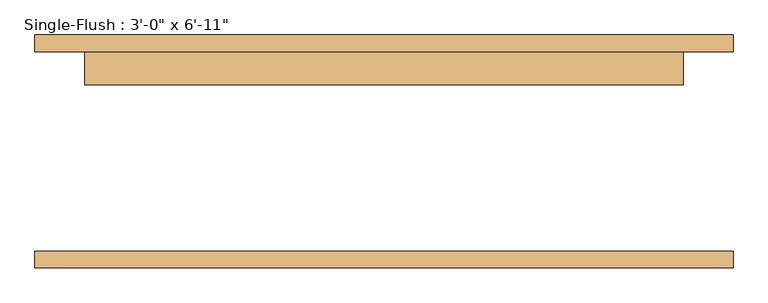
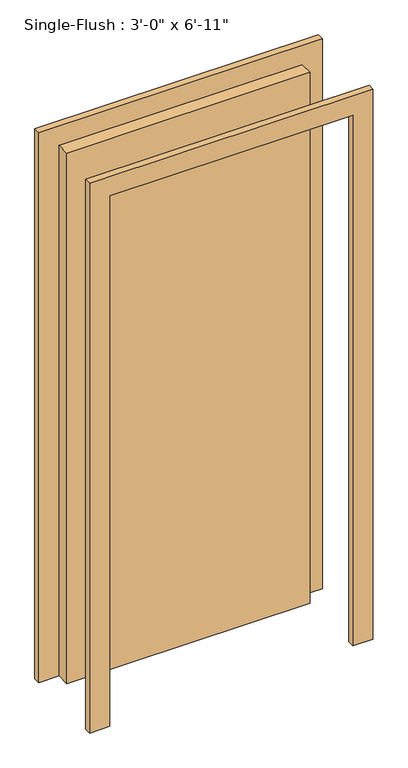
"""IFC4 building model written with IfcOpenShell, lengths in millimetres: door geometry."""

from ifc_helpers import new_model, si_unit, frame, origin, origin_with_axes, place, context, project, spatial, polyline, outline, extrude, source, transform, mapped, element, save


def door_a6ca3d0c(model_context):
    return source(origin(), model_context, "Body", "SweptSolid", [
        extrude(outline(polyline([(2184.4, -533.4), (0.0, -533.4), (0.0, -457.2), (2108.2, -457.2), (2108.2, 457.2), (0.0, 457.2), (0.0, 533.4), (2184.4, 533.4), (2184.4, -533.4)])), frame((0.0, 152.4, 0.0), z_axis=(0.0, 1.0, 0.0), x_axis=(0.0, 0.0, 1.0)), (0.0, 0.0, 1.0), 25.4),
        extrude(outline(polyline([(2184.4, 533.4), (2184.4, -533.4), (0.0, -533.4), (0.0, -457.2), (2108.2, -457.2), (2108.2, 457.2), (0.0, 457.2), (0.0, 533.4), (2184.4, 533.4)])), frame((0.0, -177.8, 0.0), z_axis=(0.0, 1.0, 0.0), x_axis=(0.0, 0.0, 1.0)), (0.0, 0.0, 1.0), 25.4),
        extrude(outline(polyline([(457.2, 101.6), (-457.2, 101.6), (-457.2, 152.4), (457.2, 152.4), (457.2, 101.6)])), origin_with_axes(), (0.0, 0.0, 1.0), 2108.2),
    ])


if __name__ == "__main__":
    model = new_model("IFC4")
    model_context = context("Model", 3, world=origin())
    ifc_project = project(units=[si_unit("LENGTHUNIT", "METRE", prefix="MILLI")], contexts=[model_context])
    site = spatial("IfcSite", under=ifc_project)
    building = spatial("IfcBuilding", under=site)
    placement = place(None, origin())
    door_shape = door_a6ca3d0c(model_context)
    element("IfcDoor", 1, ObjectType="Single-Flush : 3'-0\" x 6'-11\"", at=placement, inside=building, context=model_context, shape_type="MappedRepresentation", body=[
        mapped(door_shape, transform((0.0, 0.0, 0.0), x_axis=(1.0, 0.0, 0.0), y_axis=(0.0, 1.0, 0.0), z_axis=(0.0, 0.0, 1.0))),
    ])
    save(model, "model.ifc")

# Revit data of these elements
# Type "Single-Flush : 3'-0\" x 6'-11\""
#   Type Mark = "10"
#   Construction Type Id = "MDOOR"
#   Assembly Code = "C1020"
#   Analytic Construction = "Metal"
#   Thickness = 0' - 2"
#   Heat Transfer Coefficient (U) = 3.7021 W/(m²·K)
#   Height = 6' - 11"
#   Trim Projection Ext = 0' - 1"
#   Trim Projection Int = 0' - 1"
#   Trim Width = 0' - 3"
#   Width = 3' - 0"
#   Door Material = Door - Panel
#   Frame Material = Door - Frame
#   Visual Light Transmittance = 0
#   Solar Heat Gain Coefficient = 0
#   Function = (empty or 0)
#   Wall Closure = (empty or 0)
# Element 1 (IfcDoor, "Single-Flush : 3'-0\" x 6'-11\"")
#   Materials on its faces: "Door - Frame", "Door - Panel"
# Materials
#   "Door - Panel": class "Wood", colour RGB 210 159 95, transparency 0, Cost = 0
#   "Door - Frame": class "Miscellaneous", colour RGB 118 70 51, transparency 0, Cost = 0
